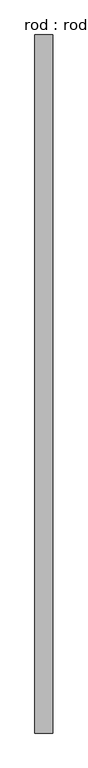
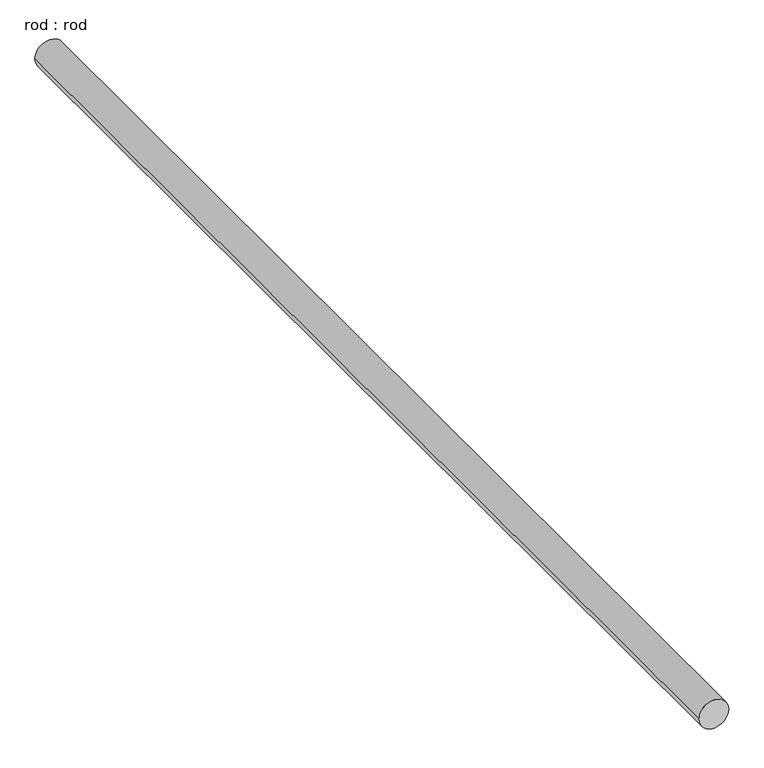
"""IFC4 building model written with IfcOpenShell, lengths in millimetres: proxy geometry, rod : rod."""

from ifc_helpers import new_model, si_unit, point, frame, frame_2d, origin, place, context, project, spatial, circle_curve, trimmed, segment, composite_curve, outline, extrude, source, transform, mapped, element, save


def rod_rod_63d51a2c(model_context):
    return source(origin(), model_context, "Body", "SweptSolid", [
        extrude(outline(composite_curve([segment(trimmed(circle_curve(frame_2d((0.0108462, 0.0)), 200.0), [point((0.0108462, 200.0))], [point((0.0108462, -200.0))], False, "CARTESIAN"), True, "CONTINUOUS"), segment(trimmed(circle_curve(frame_2d((0.0108462, 0.0)), 200.0), [point((0.0108462, -200.0))], [point((0.0108462, 200.0))], False, "CARTESIAN"), True, "CONTINUOUS")], self_intersect=False)), frame((0.0, -3626.6771394, 0.0), z_axis=(0.0, 1.0, 0.0), x_axis=(0.0, 0.0, 1.0)), (0.0, 0.0, 1.0), 15438.8115095),
    ])


if __name__ == "__main__":
    model = new_model("IFC4")
    model_context = context("Model", 3, world=origin())
    ifc_project = project(units=[si_unit("LENGTHUNIT", "METRE", prefix="MILLI")], contexts=[model_context])
    site = spatial("IfcSite", under=ifc_project)
    building = spatial("IfcBuilding", under=site)
    placement = place(None, origin())
    rod_rod_shape = rod_rod_63d51a2c(model_context)
    element("IfcBuildingElementProxy", 1, Name="rod : rod", ObjectType="rod : rod", at=placement, inside=building, context=model_context, shape_type="MappedRepresentation", body=[
        mapped(rod_rod_shape, transform((0.0, 0.0, 0.0), x_axis=(1.0, 0.0, 0.0), y_axis=(0.0, 1.0, 0.0), z_axis=(0.0, 0.0, 1.0))),
    ])
    save(model, "model.ifc")

# Revit data of these elements
# Type "rod : rod"
#   Default Elevation = 0
